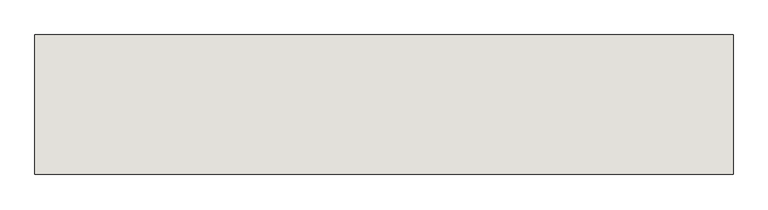
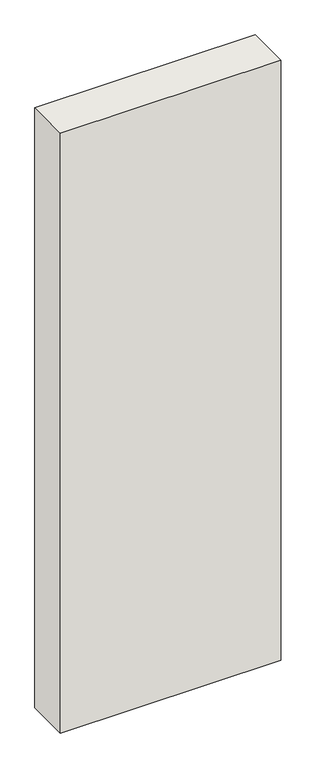
"""IFC4 building model written with IfcOpenShell, lengths in millimetres: wall geometry, Holzwand."""

import ifcopenshell
import ifcopenshell.guid

model = None  # the IFC model being written
_history = None  # IfcOwnerHistory: only IFC2X3 demands one
_inside = {}  # id of a spatial element -> (the spatial element, [elements in it])
_under = {}  # id of a project, library or spatial element -> (it, [spatial elements below it])
_declared = {}  # id of a project -> (the project, [libraries it declares])
_typed = {}  # id of a type object -> (the type object, [elements of that type])
_made_of = {}  # id of a material, layer set ... -> (it, [elements and type objects made of it])


def new_model(schema):
    """Start an empty IFC model of exactly this schema.

    Asked for "IFC4X3", IfcOpenShell would pick the latest addendum, in which some entities
    have other attributes; the version numbers below select the first issue.
    IFC2X3 requires an IfcOwnerHistory on every rooted entity: one is made here for all.
    """
    global model, _history
    if schema == "IFC4X3":
        model = ifcopenshell.file(schema_version=(4, 3, 0, 0))
    else:
        model = ifcopenshell.file(schema=schema)
    _inside.clear()
    _under.clear()
    _declared.clear()
    _typed.clear()
    _made_of.clear()
    _history = None
    if model.schema == "IFC2X3":
        org = make("IfcOrganization", Name="unknown")
        user = make(
            "IfcPersonAndOrganization",
            ThePerson=make("IfcPerson", FamilyName="unknown"),
            TheOrganization=org,
        )
        app = make(
            "IfcApplication",
            ApplicationDeveloper=org,
            Version="unknown",
            ApplicationFullName="unknown",
            ApplicationIdentifier="unknown",
        )
        _history = make(
            "IfcOwnerHistory",
            OwningUser=user,
            OwningApplication=app,
            ChangeAction="ADDED",
            CreationDate=0,
        )
    return model


def make(cls, **values):
    """One entity of the class cls with the attributes given. An attribute that is None is left unset."""
    return model.create_entity(
        cls, **{name: value for name, value in values.items() if value is not None}
    )


def rooted(cls, **values):
    """An entity with a GlobalId (a new one), such as an element, a storey or a relation."""
    return make(cls, GlobalId=ifcopenshell.guid.new(), OwnerHistory=_history, **values)


def si_unit(unit_type, name, prefix=None):
    """IfcSIUnit, for example si_unit("LENGTHUNIT", "METRE", prefix="MILLI")."""
    return make("IfcSIUnit", UnitType=unit_type, Prefix=prefix, Name=name)


def assignment(units):
    """IfcUnitAssignment: the units of a project."""
    return None if units is None else make("IfcUnitAssignment", Units=units)


def point(xyz):
    """IfcCartesianPoint."""
    return None if xyz is None else make("IfcCartesianPoint", Coordinates=xyz)


def direction(xyz):
    """IfcDirection."""
    return None if xyz is None else make("IfcDirection", DirectionRatios=xyz)


def frame(location, z_axis=None, x_axis=None):
    """IfcAxis2Placement3D, a coordinate frame: its origin and axes. An axis left out is left unset."""
    return make(
        "IfcAxis2Placement3D",
        Location=point(location),
        Axis=direction(z_axis),
        RefDirection=direction(x_axis),
    )


def origin():
    """The frame at (0, 0, 0) with its axes left unset."""
    return frame((0.0, 0.0, 0.0))


def origin_with_axes():
    """The frame at (0, 0, 0) with the z axis (0, 0, 1) and the x axis (1, 0, 0) written out."""
    return frame((0.0, 0.0, 0.0), z_axis=(0.0, 0.0, 1.0), x_axis=(1.0, 0.0, 0.0))


def place(relative_to, where):
    """IfcLocalPlacement: puts the frame where relative to a parent placement (None: the world)."""
    return make(
        "IfcLocalPlacement", PlacementRelTo=relative_to, RelativePlacement=where
    )


def context(
    kind, dimensions, precision=None, world=None, true_north=None, identifier=None
):
    """IfcGeometricRepresentationContext, for example the 3D "Model" context."""
    return make(
        "IfcGeometricRepresentationContext",
        ContextIdentifier=identifier,
        ContextType=kind,
        CoordinateSpaceDimension=dimensions,
        Precision=precision,
        WorldCoordinateSystem=world,
        TrueNorth=true_north,
    )


def project(units=None, contexts=None):
    """IfcProject with its units and contexts."""
    return rooted(
        "IfcProject",
        Name="project",
        RepresentationContexts=contexts,
        UnitsInContext=assignment(units),
    )


def spatial(cls, under=None, at=None, **own):
    """A site, building, storey or space (cls), placed at a placement, below another one or the project."""
    s = rooted(cls, ObjectPlacement=at, **own)
    if under is not None:
        _under.setdefault(under.id(), (under, []))[1].append(s)
    return s


def polyline(points):
    """IfcPolyline through the points."""
    return make("IfcPolyline", Points=[point(p) for p in points])


def outline(outer, holes=None, kind="AREA"):
    """IfcArbitraryClosedProfileDef: a profile drawn as a closed curve; with holes, ...WithVoids."""
    if holes is None:
        return make("IfcArbitraryClosedProfileDef", ProfileType=kind, OuterCurve=outer)
    return make(
        "IfcArbitraryProfileDefWithVoids",
        ProfileType=kind,
        OuterCurve=outer,
        InnerCurves=holes,
    )


def extrude(swept, where, along, depth):
    """IfcExtrudedAreaSolid: the profile swept, set in the frame where, extruded along a direction by depth."""
    return make(
        "IfcExtrudedAreaSolid",
        SweptArea=swept,
        Position=where,
        ExtrudedDirection=direction(along),
        Depth=depth,
    )


def shape(context_of_items, identifier, shape_type, items):
    """IfcShapeRepresentation: the items that make up one representation, for example the "Body"."""
    return make(
        "IfcShapeRepresentation",
        ContextOfItems=context_of_items,
        RepresentationIdentifier=identifier,
        RepresentationType=shape_type,
        Items=items,
    )


def source(mapping_origin, context_of_items, identifier, shape_type, items):
    """IfcRepresentationMap: a shape defined once, which mapped items show again and again."""
    return make(
        "IfcRepresentationMap",
        MappingOrigin=mapping_origin,
        MappedRepresentation=shape(context_of_items, identifier, shape_type, items),
    )


def transform(
    local_origin,
    x_axis=None,
    y_axis=None,
    z_axis=None,
    scale=None,
    scale2=None,
    scale3=None,
    uniform=True,
):
    """IfcCartesianTransformationOperator3D, or its non-uniform kind. x_axis, y_axis, z_axis: its Axis1, 2, 3."""
    if uniform:
        return make(
            "IfcCartesianTransformationOperator3D",
            Axis1=direction(x_axis),
            Axis2=direction(y_axis),
            LocalOrigin=point(local_origin),
            Scale=scale,
            Axis3=direction(z_axis),
        )
    return make(
        "IfcCartesianTransformationOperator3DnonUniform",
        Axis1=direction(x_axis),
        Axis2=direction(y_axis),
        LocalOrigin=point(local_origin),
        Scale=scale,
        Axis3=direction(z_axis),
        Scale2=scale2,
        Scale3=scale3,
    )


def mapped(mapping_source, mapping_target):
    """IfcMappedItem: shows the shape of a source again, moved by a transform."""
    return make(
        "IfcMappedItem", MappingSource=mapping_source, MappingTarget=mapping_target
    )


def made_of(thing, what):
    """Note that an element or type object is made of a material, layer set ...; save() writes the relation."""
    if what is not None:
        _made_of.setdefault(what.id(), (what, []))[1].append(thing)
    return thing


def element(
    cls,
    number,
    at=None,
    inside=None,
    cuts=None,
    type_object=None,
    material=None,
    context=None,
    identifier="Body",
    shape_type=None,
    held_by="IfcProductDefinitionShape",
    body=None,
    shapes=None,
    **own,
):
    """One element of the class cls, such as IfcWall. Its Tag is "e" and its number.

    at: its placement. inside: the storey or other place that contains it. cuts: it is an
    opening in that element (IfcRelVoidsElement). A single representation is given by context,
    identifier, shape_type and body (its items); several are given by shapes. held_by: the class
    of the entity that holds the representations. save() writes the other relations.
    """
    e = rooted(cls, Tag="e%d" % number, ObjectPlacement=at, **own)
    if body is not None:
        shapes = [shape(context, identifier, shape_type, body)]
    if shapes is not None:
        e.Representation = make(held_by, Representations=shapes)
    if inside is not None:
        _inside.setdefault(inside.id(), (inside, []))[1].append(e)
    if cuts is not None:
        rooted(
            "IfcRelVoidsElement", RelatingBuildingElement=cuts, RelatedOpeningElement=e
        )
    if type_object is not None:
        _typed.setdefault(type_object.id(), (type_object, []))[1].append(e)
    return made_of(e, material)


def aggregate(whole, parts):
    """IfcRelAggregates: a whole, such as a stair, and the parts it consists of."""
    return rooted("IfcRelAggregates", RelatingObject=whole, RelatedObjects=parts)


def save(model, path):
    """Write the relations noted so far, then the file.

    IfcRelAggregates (storeys below a building ...), IfcRelContainedInSpatialStructure (elements
    in a storey), IfcRelDefinesByType, IfcRelAssociatesMaterial and IfcRelDeclares: one each for
    every whole, place, type object, material and project.
    """
    for whole, parts in _under.values():
        aggregate(whole, parts)
    for where, things in _inside.values():
        rooted(
            "IfcRelContainedInSpatialStructure",
            RelatedElements=things,
            RelatingStructure=where,
        )
    for kind, things in _typed.values():
        rooted("IfcRelDefinesByType", RelatedObjects=things, RelatingType=kind)
    for what, things in _made_of.values():
        rooted("IfcRelAssociatesMaterial", RelatedObjects=things, RelatingMaterial=what)
    for by, libraries in _declared.values():
        rooted("IfcRelDeclares", RelatingContext=by, RelatedDefinitions=libraries)
    model.write(path)


def wall_e4fc0cee(model_context):
    return source(origin(), model_context, "Body", "SweptSolid", [
        extrude(outline(polyline([(1001.7, 200.0), (1001.7, 0.0), (0.0, 0.0), (0.0, 200.0), (1001.7, 200.0)])), origin_with_axes(), (0.0, 0.0, 1.0), 2880.0),
    ])


if __name__ == "__main__":
    model = new_model("IFC4")
    model_context = context("Model", 3, world=origin())
    ifc_project = project(units=[si_unit("LENGTHUNIT", "METRE", prefix="MILLI")], contexts=[model_context])
    site = spatial("IfcSite", under=ifc_project)
    building = spatial("IfcBuilding", under=site)
    placement = place(None, origin())
    wall_shape = wall_e4fc0cee(model_context)
    element("IfcWall", 1, ObjectType="Holzwand", at=placement, inside=building, context=model_context, shape_type="MappedRepresentation", body=[
        mapped(wall_shape, transform((0.0, 0.0, 0.0), x_axis=(1.0, 0.0, 0.0), y_axis=(0.0, 1.0, 0.0), z_axis=(0.0, 0.0, 1.0))),
    ])
    save(model, "model.ifc")

# Revit data of these elements
# Element 1 (IfcWall, "Holzwand")
#   Materials on its faces: "holzschalung"
# Materials
#   "holzschalung": class "Unassigned", colour RGB 128 128 128, transparency 0
